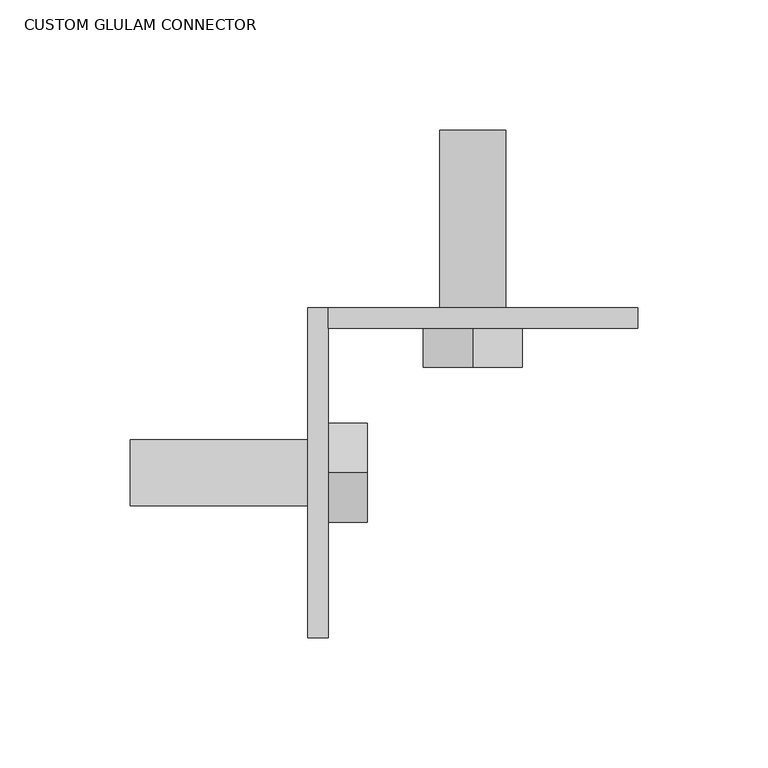
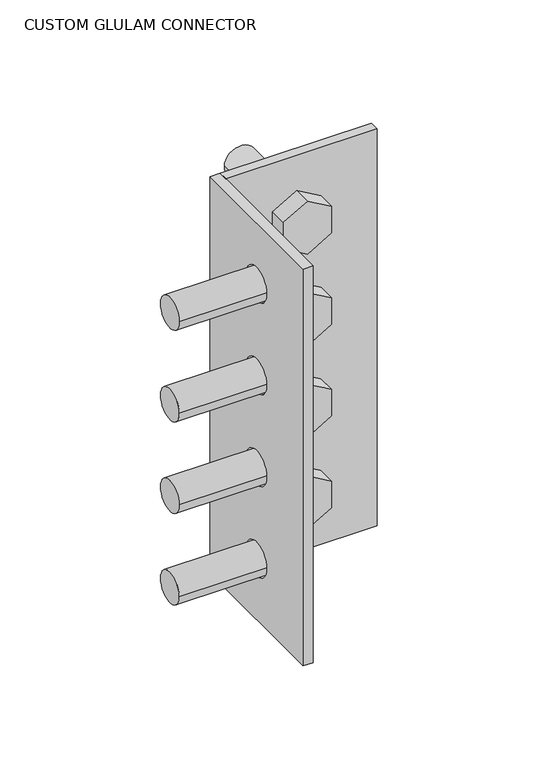
"""IFC4 building model written with IfcOpenShell, lengths in millimetres: fastener geometry, CUSTOM GLULAM CONNECTOR."""

from ifc_helpers import new_model, si_unit, point, frame, frame_2d, origin, place, context, project, spatial, polyline, circle_curve, trimmed, segment, composite_curve, outline, extrude, source, transform, mapped, element, save
from ifc_brep_helpers import plane_surface, revolved_surface, advanced_brep


def custom_glulam_connector_0c2b97b1(model_context):
    return source(origin(), model_context, "Body", "SolidModel", [
        extrude(outline(polyline([(719.1375, 214.3125), (719.1375, 95.25), (388.9375, 95.25), (388.9375, 214.3125), (719.1375, 214.3125)]), holes=[composite_curve([segment(trimmed(circle_curve(frame_2d((668.3375, 150.8125)), 13.890625), [point((668.3375, 164.703125))], [point((668.3375, 136.921875))], True, "CARTESIAN"), True, "CONTINUOUS"), segment(trimmed(circle_curve(frame_2d((668.3375, 150.8125)), 13.890625), [point((668.3375, 136.921875))], [point((668.3375, 164.703125))], True, "CARTESIAN"), True, "CONTINUOUS")], self_intersect=False), composite_curve([segment(trimmed(circle_curve(frame_2d((592.1375, 150.8125)), 13.890625), [point((592.1375, 164.703125))], [point((592.1375, 136.921875))], True, "CARTESIAN"), True, "CONTINUOUS"), segment(trimmed(circle_curve(frame_2d((592.1375, 150.8125)), 13.890625), [point((592.1375, 136.921875))], [point((592.1375, 164.703125))], True, "CARTESIAN"), True, "CONTINUOUS")], self_intersect=False), composite_curve([segment(trimmed(circle_curve(frame_2d((515.9375, 150.8125)), 13.890625), [point((515.9375, 164.703125))], [point((515.9375, 136.921875))], True, "CARTESIAN"), True, "CONTINUOUS"), segment(trimmed(circle_curve(frame_2d((515.9375, 150.8125)), 13.890625), [point((515.9375, 136.921875))], [point((515.9375, 164.703125))], True, "CARTESIAN"), True, "CONTINUOUS")], self_intersect=False), composite_curve([segment(trimmed(circle_curve(frame_2d((439.7375, 150.8125)), 13.890625), [point((439.7375, 164.703125))], [point((439.7375, 136.921875))], True, "CARTESIAN"), True, "CONTINUOUS"), segment(trimmed(circle_curve(frame_2d((439.7375, 150.8125)), 13.890625), [point((439.7375, 136.921875))], [point((439.7375, 164.703125))], True, "CARTESIAN"), True, "CONTINUOUS")], self_intersect=False)]), frame((0.0, 55.5625, 0.0), z_axis=(0.0, 1.0, 0.0), x_axis=(0.0, 0.0, 1.0)), (0.0, 0.0, 1.0), 7.9375),
        extrude(outline(polyline([(679.3360226, 131.7625), (657.3389774, 131.7625), (646.3404547, 150.8125), (657.3389774, 169.8625), (679.3360226, 169.8625), (690.3345453, 150.8125), (679.3360226, 131.7625)])), frame((0.0, 40.5804688, 0.0), z_axis=(0.0, 1.0, 0.0), x_axis=(0.0, 0.0, 1.0)), (0.0, 0.0, 1.0), 14.9820312),
        extrude(outline(composite_curve([segment(trimmed(circle_curve(frame_2d((668.3375, 150.8125)), 12.7), [point((668.3375, 138.1125))], [point((668.3375, 163.5125))], False, "CARTESIAN"), True, "CONTINUOUS"), segment(trimmed(circle_curve(frame_2d((668.3375, 150.8125)), 12.7), [point((668.3375, 163.5125))], [point((668.3375, 138.1125))], False, "CARTESIAN"), True, "CONTINUOUS")], self_intersect=False)), frame((0.0, 55.5625, 0.0), z_axis=(0.0, 1.0, 0.0), x_axis=(0.0, 0.0, 1.0)), (0.0, 0.0, 1.0), 76.2),
        extrude(outline(polyline([(603.1360226, 131.7625), (581.1389774, 131.7625), (570.1404547, 150.8125), (581.1389774, 169.8625), (603.1360226, 169.8625), (614.1345453, 150.8125), (603.1360226, 131.7625)])), frame((0.0, 40.5804688, 0.0), z_axis=(0.0, 1.0, 0.0), x_axis=(0.0, 0.0, 1.0)), (0.0, 0.0, 1.0), 14.9820312),
        extrude(outline(composite_curve([segment(trimmed(circle_curve(frame_2d((592.1375, 150.8125)), 12.7), [point((592.1375, 138.1125))], [point((592.1375, 163.5125))], False, "CARTESIAN"), True, "CONTINUOUS"), segment(trimmed(circle_curve(frame_2d((592.1375, 150.8125)), 12.7), [point((592.1375, 163.5125))], [point((592.1375, 138.1125))], False, "CARTESIAN"), True, "CONTINUOUS")], self_intersect=False)), frame((0.0, 55.5625, 0.0), z_axis=(0.0, 1.0, 0.0), x_axis=(0.0, 0.0, 1.0)), (0.0, 0.0, 1.0), 76.2),
        extrude(outline(polyline([(679.3360226, 131.7625), (657.3389774, 131.7625), (646.3404547, 150.8125), (657.3389774, 169.8625), (679.3360226, 169.8625), (690.3345453, 150.8125), (679.3360226, 131.7625)])), frame((0.0, 40.5804688, 0.0), z_axis=(0.0, 1.0, 0.0), x_axis=(0.0, 0.0, 1.0)), (0.0, 0.0, 1.0), 14.9820312),
        extrude(outline(composite_curve([segment(trimmed(circle_curve(frame_2d((668.3375, 150.8125)), 12.7), [point((668.3375, 138.1125))], [point((668.3375, 163.5125))], False, "CARTESIAN"), True, "CONTINUOUS"), segment(trimmed(circle_curve(frame_2d((668.3375, 150.8125)), 12.7), [point((668.3375, 163.5125))], [point((668.3375, 138.1125))], False, "CARTESIAN"), True, "CONTINUOUS")], self_intersect=False)), frame((0.0, 55.5625, 0.0), z_axis=(0.0, 1.0, 0.0), x_axis=(0.0, 0.0, 1.0)), (0.0, 0.0, 1.0), 76.2),
        extrude(outline(polyline([(526.9360226, 131.7625), (504.9389774, 131.7625), (493.9404547, 150.8125), (504.9389774, 169.8625), (526.9360226, 169.8625), (537.9345453, 150.8125), (526.9360226, 131.7625)])), frame((0.0, 40.5804688, 0.0), z_axis=(0.0, 1.0, 0.0), x_axis=(0.0, 0.0, 1.0)), (0.0, 0.0, 1.0), 14.9820312),
        extrude(outline(composite_curve([segment(trimmed(circle_curve(frame_2d((515.9375, 150.8125)), 12.7), [point((515.9375, 138.1125))], [point((515.9375, 163.5125))], False, "CARTESIAN"), True, "CONTINUOUS"), segment(trimmed(circle_curve(frame_2d((515.9375, 150.8125)), 12.7), [point((515.9375, 163.5125))], [point((515.9375, 138.1125))], False, "CARTESIAN"), True, "CONTINUOUS")], self_intersect=False)), frame((0.0, 55.5625, 0.0), z_axis=(0.0, 1.0, 0.0), x_axis=(0.0, 0.0, 1.0)), (0.0, 0.0, 1.0), 76.2),
        extrude(outline(polyline([(450.7360226, 131.7625), (428.7389774, 131.7625), (417.7404547, 150.8125), (428.7389774, 169.8625), (450.7360226, 169.8625), (461.7345453, 150.8125), (450.7360226, 131.7625)])), frame((0.0, 40.5804688, 0.0), z_axis=(0.0, 1.0, 0.0), x_axis=(0.0, 0.0, 1.0)), (0.0, 0.0, 1.0), 14.9820312),
        extrude(outline(composite_curve([segment(trimmed(circle_curve(frame_2d((439.7375, 150.8125)), 12.7), [point((439.7375, 138.1125))], [point((439.7375, 163.5125))], False, "CARTESIAN"), True, "CONTINUOUS"), segment(trimmed(circle_curve(frame_2d((439.7375, 150.8125)), 12.7), [point((439.7375, 163.5125))], [point((439.7375, 138.1125))], False, "CARTESIAN"), True, "CONTINUOUS")], self_intersect=False)), frame((0.0, 55.5625, 0.0), z_axis=(0.0, 1.0, 0.0), x_axis=(0.0, 0.0, 1.0)), (0.0, 0.0, 1.0), 76.2),
        advanced_brep(
        [(95.25, 13.890625, 592.1375), (95.25, -13.890625, 592.1375), (87.3125, -13.890625, 592.1375), (87.3125, 13.890625, 592.1375), (95.25, 63.5, 719.1375), (87.3125, 63.5, 719.1375), (87.3125, -63.5, 719.1375), (95.25, -63.5, 719.1375), (95.25, 55.5625, 719.1375), (87.3125, 63.5, 388.9375), (87.3125, -63.5, 388.9375), (87.3125, 13.890625, 668.3375), (87.3125, -13.890625, 668.3375), (87.3125, 13.890625, 515.9375), (87.3125, -13.890625, 515.9375), (87.3125, 13.890625, 439.7375), (87.3125, -13.890625, 439.7375), (95.25, -63.5, 388.9375), (95.25, 55.5625, 388.9375), (95.25, 63.5, 388.9375), (95.25, -13.890625, 668.3375), (95.25, 13.890625, 668.3375), (95.25, -13.890625, 515.9375), (95.25, 13.890625, 515.9375), (95.25, -13.890625, 439.7375), (95.25, 13.890625, 439.7375)],
        [
            (0, 1, circle_curve(frame((95.25, 0.0, 592.1375), z_axis=(1.0, 0.0, 0.0), x_axis=(0.0, -1.0, 0.0)), 13.890625)),
            (1, 2),
            (2, 3, circle_curve(frame((87.3125, 0.0, 592.1375), z_axis=(-1.0, 0.0, 0.0), x_axis=(0.0, -1.0, 0.0)), 13.890625)),
            (3, 0),
            (4, 5),
            (5, 6),
            (6, 7),
            (7, 8),
            (8, 4),
            (5, 9),
            (9, 10),
            (10, 6),
            (11, 12, circle_curve(frame((87.3125, 0.0, 668.3375), z_axis=(1.0, 0.0, 0.0), x_axis=(0.0, -1.0, 0.0)), 13.890625)),
            (12, 11, circle_curve(frame((87.3125, 0.0, 668.3375), z_axis=(1.0, 0.0, 0.0), x_axis=(0.0, -1.0, 0.0)), 13.890625)),
            (2, 3, circle_curve(frame((87.3125, 0.0, 592.1375), z_axis=(1.0, 0.0, 0.0), x_axis=(0.0, -1.0, 0.0)), 13.890625)),
            (13, 14, circle_curve(frame((87.3125, 0.0, 515.9375), z_axis=(1.0, 0.0, 0.0), x_axis=(0.0, -1.0, 0.0)), 13.890625)),
            (14, 13, circle_curve(frame((87.3125, 0.0, 515.9375), z_axis=(1.0, 0.0, 0.0), x_axis=(0.0, -1.0, 0.0)), 13.890625)),
            (15, 16, circle_curve(frame((87.3125, 0.0, 439.7375), z_axis=(1.0, 0.0, 0.0), x_axis=(0.0, -1.0, 0.0)), 13.890625)),
            (16, 15, circle_curve(frame((87.3125, 0.0, 439.7375), z_axis=(1.0, 0.0, 0.0), x_axis=(0.0, -1.0, 0.0)), 13.890625)),
            (7, 17),
            (17, 18),
            (18, 19),
            (19, 4),
            (20, 21, circle_curve(frame((95.25, 0.0, 668.3375), z_axis=(-1.0, 0.0, 0.0), x_axis=(0.0, -1.0, 0.0)), 13.890625)),
            (21, 20, circle_curve(frame((95.25, 0.0, 668.3375), z_axis=(-1.0, 0.0, 0.0), x_axis=(0.0, -1.0, 0.0)), 13.890625)),
            (0, 1, circle_curve(frame((95.25, 0.0, 592.1375), z_axis=(-1.0, 0.0, 0.0), x_axis=(0.0, -1.0, 0.0)), 13.890625)),
            (22, 23, circle_curve(frame((95.25, 0.0, 515.9375), z_axis=(-1.0, 0.0, 0.0), x_axis=(0.0, -1.0, 0.0)), 13.890625)),
            (23, 22, circle_curve(frame((95.25, 0.0, 515.9375), z_axis=(-1.0, 0.0, 0.0), x_axis=(0.0, -1.0, 0.0)), 13.890625)),
            (24, 25, circle_curve(frame((95.25, 0.0, 439.7375), z_axis=(-1.0, 0.0, 0.0), x_axis=(0.0, -1.0, 0.0)), 13.890625)),
            (25, 24, circle_curve(frame((95.25, 0.0, 439.7375), z_axis=(-1.0, 0.0, 0.0), x_axis=(0.0, -1.0, 0.0)), 13.890625)),
            (19, 9),
            (10, 17),
            (12, 20),
            (21, 11),
            (22, 14),
            (13, 23),
            (24, 16),
            (15, 25),
        ],
        [
            revolved_surface(polyline([(95.25, -13.890625, 592.1375), (87.3125, -13.890625, 592.1375)]), (87.3125, 0.0, 592.1375), (1.0, 0.0, 0.0)),
            plane_surface(frame((95.25, -63.5, 719.1375), z_axis=(0.0, 0.0, 1.0), x_axis=(-1.0, 0.0, 0.0))),
            plane_surface(frame((87.3125, 63.5, 719.1375), z_axis=(-1.0, 0.0, 0.0), x_axis=(0.0, -1.0, 0.0))),
            plane_surface(frame((95.25, 63.5, 719.1375), z_axis=(1.0, 0.0, 0.0), x_axis=(0.0, 1.0, 0.0))),
            plane_surface(frame((95.25, 63.5, 719.1375), z_axis=(0.0, 1.0, 0.0), x_axis=(-1.0, 0.0, 0.0))),
            plane_surface(frame((95.25, -63.5, 388.9375), z_axis=(0.0, -1.0, 0.0), x_axis=(-1.0, 0.0, 0.0))),
            revolved_surface(polyline([(95.25, -13.890625, 668.3375), (87.3125, -13.890625, 668.3375)]), (87.3125, 0.0, 668.3375), (1.0, 0.0, 0.0)),
            plane_surface(frame((95.25, 63.5, 388.9375), z_axis=(0.0, 0.0, -1.0), x_axis=(-1.0, 0.0, 0.0))),
            revolved_surface(polyline([(95.25, -13.890625, 515.9375), (87.3125, -13.890625, 515.9375)]), (87.3125, 0.0, 515.9375), (1.0, 0.0, 0.0)),
            revolved_surface(polyline([(95.25, -13.890625, 439.7375), (87.3125, -13.890625, 439.7375)]), (87.3125, 0.0, 439.7375), (1.0, 0.0, 0.0)),
        ],
        [
            (0, [[1, 2, 3, 4]]),
            (1, [[5, 6, 7, 8, 9]]),
            (2, [[-6, 10, 11, 12], [13, 14], [-3, 15], [16, 17], [18, 19]]),
            (3, [[20, 21, 22, 23, -9, -8], [24, 25], [-1, 26], [27, 28], [29, 30]]),
            (4, [[31, -10, -5, -23]]),
            (5, [[-7, -12, 32, -20]]),
            (6, [[-14, 33, -25, 34]]),
            (6, [[-24, -33, -13, -34]]),
            (0, [[-15, -2, -26, -4]]),
            (7, [[-32, -11, -31, -22, -21]]),
            (8, [[-27, 35, -16, 36]]),
            (9, [[-29, 37, -18, 38]]),
            (9, [[-19, -37, -30, -38]]),
            (8, [[-17, -35, -28, -36]]),
        ],
    ),
        extrude(outline(polyline([(19.05, 679.3360226), (19.05, 657.3389774), (0.0, 646.3404547), (-19.05, 657.3389774), (-19.05, 679.3360226), (0.0, 690.3345453), (19.05, 679.3360226)])), frame((95.25, 0.0, 0.0), z_axis=(1.0, 0.0, 0.0), x_axis=(0.0, 1.0, 0.0)), (0.0, 0.0, 1.0), 14.9820312),
        extrude(outline(composite_curve([segment(trimmed(circle_curve(frame_2d((0.0, 668.3375)), 12.7), [point((12.7, 668.3375))], [point((-12.7, 668.3375))], False, "CARTESIAN"), True, "CONTINUOUS"), segment(trimmed(circle_curve(frame_2d((0.0, 668.3375)), 12.7), [point((-12.7, 668.3375))], [point((12.7, 668.3375))], False, "CARTESIAN"), True, "CONTINUOUS")], self_intersect=False)), frame((19.05, 0.0, 0.0), z_axis=(1.0, 0.0, 0.0), x_axis=(0.0, 1.0, 0.0)), (0.0, 0.0, 1.0), 76.2),
        extrude(outline(polyline([(19.05, 603.1360226), (19.05, 581.1389774), (0.0, 570.1404547), (-19.05, 581.1389774), (-19.05, 603.1360226), (0.0, 614.1345453), (19.05, 603.1360226)])), frame((95.25, 0.0, 0.0), z_axis=(1.0, 0.0, 0.0), x_axis=(0.0, 1.0, 0.0)), (0.0, 0.0, 1.0), 14.9820312),
        extrude(outline(composite_curve([segment(trimmed(circle_curve(frame_2d((0.0, 592.1375)), 12.7), [point((12.7, 592.1375))], [point((-12.7, 592.1375))], False, "CARTESIAN"), True, "CONTINUOUS"), segment(trimmed(circle_curve(frame_2d((0.0, 592.1375)), 12.7), [point((-12.7, 592.1375))], [point((12.7, 592.1375))], False, "CARTESIAN"), True, "CONTINUOUS")], self_intersect=False)), frame((19.05, 0.0, 0.0), z_axis=(1.0, 0.0, 0.0), x_axis=(0.0, 1.0, 0.0)), (0.0, 0.0, 1.0), 76.2),
        extrude(outline(polyline([(19.05, 679.3360226), (19.05, 657.3389774), (0.0, 646.3404547), (-19.05, 657.3389774), (-19.05, 679.3360226), (0.0, 690.3345453), (19.05, 679.3360226)])), frame((95.25, 0.0, 0.0), z_axis=(1.0, 0.0, 0.0), x_axis=(0.0, 1.0, 0.0)), (0.0, 0.0, 1.0), 14.9820312),
        extrude(outline(composite_curve([segment(trimmed(circle_curve(frame_2d((0.0, 668.3375)), 12.7), [point((12.7, 668.3375))], [point((-12.7, 668.3375))], False, "CARTESIAN"), True, "CONTINUOUS"), segment(trimmed(circle_curve(frame_2d((0.0, 668.3375)), 12.7), [point((-12.7, 668.3375))], [point((12.7, 668.3375))], False, "CARTESIAN"), True, "CONTINUOUS")], self_intersect=False)), frame((19.05, 0.0, 0.0), z_axis=(1.0, 0.0, 0.0), x_axis=(0.0, 1.0, 0.0)), (0.0, 0.0, 1.0), 76.2),
        extrude(outline(polyline([(19.05, 526.9360226), (19.05, 504.9389774), (0.0, 493.9404547), (-19.05, 504.9389774), (-19.05, 526.9360226), (0.0, 537.9345453), (19.05, 526.9360226)])), frame((95.25, 0.0, 0.0), z_axis=(1.0, 0.0, 0.0), x_axis=(0.0, 1.0, 0.0)), (0.0, 0.0, 1.0), 14.9820312),
        extrude(outline(composite_curve([segment(trimmed(circle_curve(frame_2d((0.0, 515.9375)), 12.7), [point((12.7, 515.9375))], [point((-12.7, 515.9375))], False, "CARTESIAN"), True, "CONTINUOUS"), segment(trimmed(circle_curve(frame_2d((0.0, 515.9375)), 12.7), [point((-12.7, 515.9375))], [point((12.7, 515.9375))], False, "CARTESIAN"), True, "CONTINUOUS")], self_intersect=False)), frame((19.05, 0.0, 0.0), z_axis=(1.0, 0.0, 0.0), x_axis=(0.0, 1.0, 0.0)), (0.0, 0.0, 1.0), 76.2),
        extrude(outline(polyline([(19.05, 450.7360226), (19.05, 428.7389774), (0.0, 417.7404547), (-19.05, 428.7389774), (-19.05, 450.7360226), (0.0, 461.7345453), (19.05, 450.7360226)])), frame((95.25, 0.0, 0.0), z_axis=(1.0, 0.0, 0.0), x_axis=(0.0, 1.0, 0.0)), (0.0, 0.0, 1.0), 14.9820312),
        extrude(outline(composite_curve([segment(trimmed(circle_curve(frame_2d((0.0, 439.7375)), 12.7), [point((12.7, 439.7375))], [point((-12.7, 439.7375))], False, "CARTESIAN"), True, "CONTINUOUS"), segment(trimmed(circle_curve(frame_2d((0.0, 439.7375)), 12.7), [point((-12.7, 439.7375))], [point((12.7, 439.7375))], False, "CARTESIAN"), True, "CONTINUOUS")], self_intersect=False)), frame((19.05, 0.0, 0.0), z_axis=(1.0, 0.0, 0.0), x_axis=(0.0, 1.0, 0.0)), (0.0, 0.0, 1.0), 76.2),
    ])


if __name__ == "__main__":
    model = new_model("IFC4")
    model_context = context("Model", 3, world=origin())
    ifc_project = project(units=[si_unit("LENGTHUNIT", "METRE", prefix="MILLI")], contexts=[model_context])
    site = spatial("IfcSite", under=ifc_project)
    building = spatial("IfcBuilding", under=site)
    placement = place(None, origin())
    custom_glulam_connector_shape = custom_glulam_connector_0c2b97b1(model_context)
    element("IfcFastener", 1, ObjectType="CUSTOM GLULAM CONNECTOR : CUSTOM - L5\"x5\"x5/16\"x13\" - HDG", at=placement, inside=building, context=model_context, shape_type="MappedRepresentation", body=[
        mapped(custom_glulam_connector_shape, transform((0.0, 0.0, 0.0), x_axis=(1.0, 0.0, 0.0), y_axis=(0.0, 1.0, 0.0), z_axis=(0.0, 0.0, 1.0))),
    ])
    save(model, "model.ifc")

# Revit data of these elements
# Type "CUSTOM GLULAM CONNECTOR : CUSTOM - L5\"x5\"x5/16\"x13\" - HDG"
#   Width - Top = 0' - 6 7/8"
#   Top/Bottom Plate Thickness = 0' - 0 5/16"
#   Top/Bottom Plate - Width = 0' - 7 1/2"
#   Rod Radius = 0' - 0 1/2"
#   Rod Length [instance default] = 1' - 0"
#   Plate Thickness = 0' - 0 5/16"
#   Offset - Upper Plate 2 = 0' - 0"
#   Height of Plate = 1' - 3"
#   Width - Bottom = 0' - 6 7/8"
#   Plate Width = 0' - 5"
#   Bracket Width = 0' - 5 1/4"
#   Bracket Thickness = 0' - 0 5/8"
#   Bracket Offset in X = 0' - 3 3/4"
#   Bracket Offset in Y = 0' - 0 3/4"
#   Bracket Offset = 0' - 1 1/2"
#   Bracket Leg = 0' - 8"
#   Bracket Hole Radius - Up = 0' - 0 1/2"
#   Bracket Hole Radius - Down = 0' - 0 1/2"
#   Bracket Hole Offset = 0' - 2"
#   Beam Width = 0' - 7 3/8"
#   Angle 2 = 61.00°
#   Angle 1 = 151.00°
#   Top Plate Visible = no
#   Rod Visibility = no
#   Plate Visibility - Upper Right 2 = yes
#   Plate Visibility - Upper Right 1 = yes
#   Plate Visibility - Upper Left 2 = no
#   Plate Visibility - Upper Left 1 = no
#   Plate Visibility - Lower Right 2 = no
#   Plate Visibility - Lower Right 1 = no
#   Plate Visibility - Lower Left 2 = no
#   Plate Visibility - Lower Left 1 = no
#   Bracket Visibility = no
#   Bottom Plate Visible = no
#   Upper Plates - 2 = element 1868899
#   Upper Plates - 1 = element 1868901
#   Lower Plates = element 1746392
#   Bracket Material = L5"x5"x5/16" STEEL ANGLE (HDG AFTER FABRICATION)
#   URL = ""
# Element 1 (IfcFastener, "CUSTOM GLULAM CONNECTOR : CUSTOM - L5\"x5\"x5/16\"x13\" - HDG")
#   Materials on its faces: "1\" GALV. LAG BOLT (LENGTH = 1/2\" SHY OF GLULAM DEPTH) -  (GALV. THRU BOLT IF PLATE ON OPP. SIDE OF STRUCT MEMBER)", "L5\"x5\"x5/16\" STEEL ANGLE (HDG AFTER FABRICATION)"
# Materials
#   "L5\"x5\"x5/16\" STEEL ANGLE (HDG AFTER FABRICATION)": class "Generic", colour RGB 232 232 232, transparency 0, Cost = 0
#   "1\" GALV. LAG BOLT (LENGTH = 1/2\" SHY OF GLULAM DEPTH) -  (GALV. THRU BOLT IF PLATE ON OPP. SIDE OF STRUCT MEMBER)": class "Generic", colour RGB 120 120 120, transparency 0, Cost = 0
